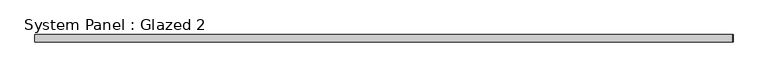
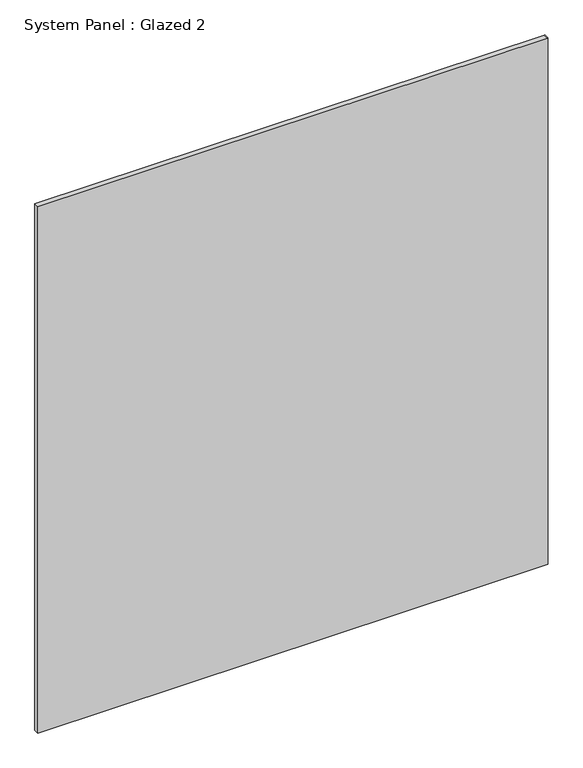
"""IFC4 building model written with IfcOpenShell, lengths in millimetres: plate geometry, System Panel : Glazed 2."""

from ifc_helpers import new_model, si_unit, frame, origin, place, context, project, spatial, polyline, outline, extrude, source, transform, mapped, element, save


def system_panel_glazed_2_d2c927cb(model_context):
    return source(origin(), model_context, "Body", "SweptSolid", [
        extrude(outline(polyline([(0.0, -1236.5882317), (0.0, 1236.5882317), (2695.2, 1236.5882317), (2695.2, 1234.6897061), (2695.2, -1236.5882317), (0.0, -1236.5882317)])), frame((0.0, -44.45, 0.0), z_axis=(0.0, 1.0, 0.0), x_axis=(0.0, 0.0, 1.0)), (0.0, 0.0, 1.0), 25.4),
    ])


if __name__ == "__main__":
    model = new_model("IFC4")
    model_context = context("Model", 3, world=origin())
    ifc_project = project(units=[si_unit("LENGTHUNIT", "METRE", prefix="MILLI")], contexts=[model_context])
    site = spatial("IfcSite", under=ifc_project)
    building = spatial("IfcBuilding", under=site)
    placement = place(None, origin())
    system_panel_glazed_2_shape = system_panel_glazed_2_d2c927cb(model_context)
    element("IfcPlate", 1, ObjectType="System Panel : Glazed 2", at=placement, inside=building, context=model_context, shape_type="MappedRepresentation", body=[
        mapped(system_panel_glazed_2_shape, transform((0.0, 0.0, 0.0), x_axis=(1.0, 0.0, 0.0), y_axis=(0.0, 1.0, 0.0), z_axis=(0.0, 0.0, 1.0))),
    ])
    save(model, "model.ifc")

# Revit data of these elements
# Element 1 (IfcPlate, "System Panel : Glazed 2")
#   Materials on its faces: "Glass, Clear Glazing"
# Materials
#   "Glass, Clear Glazing": class "Glass", colour RGB 213 204 197, transparency 0.85, Description = "Clear glazing", Cost = 0
